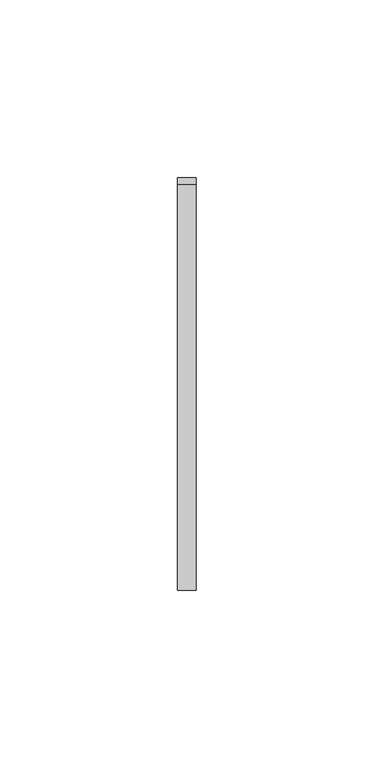
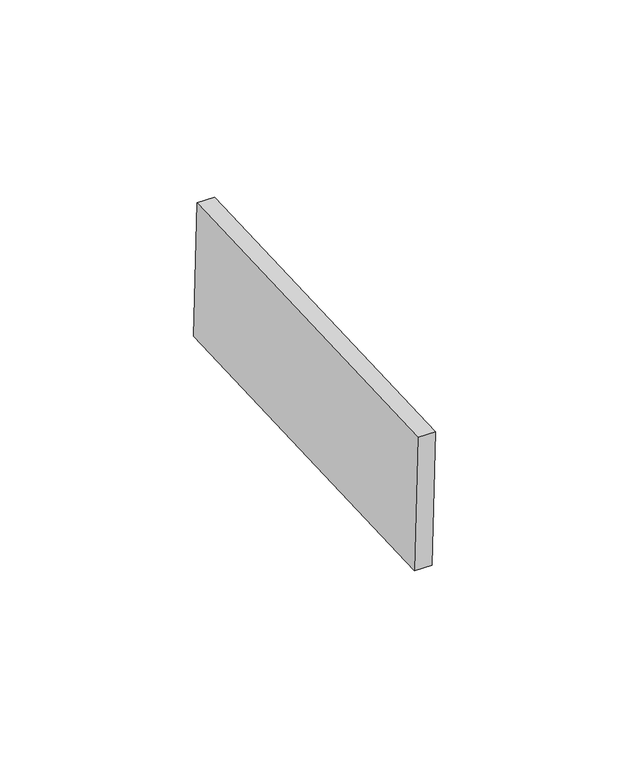
"""IFC4 building model written with IfcOpenShell, lengths in millimetres: proxy geometry, Inner panel:Inner panel:1:Inner panel:1 : Inner panel:Inner panel:300324:2:Inner panel:1:Inner panel:1 : Inner panel:Inner panel:300324:2 : Inner panel:Inner panel:1:Inner panel:1 : Inner panel:Inner panel:300324:300043:84 : Inner panel:Inner panel:1:Inner panel:1 : Inner panel:Inner panel:300324:2:Inner panel:1:Inner panel:1 : Inner panel:Inner panel:300324:2 : Inner panel:Inner panel:1:Inner panel:1 : Inner panel:Inner panel:300324:300043:308120."""

from ifc_helpers import new_model, si_unit, frame, origin, place, context, project, spatial, polyline, outline, extrude, source, transform, mapped, element, save


def generic_models_0b559e5c(model_context):
    return source(origin(), model_context, "Body", "SweptSolid", [
        extrude(outline(polyline([(0.0, -114.2999999), (0.0, 0.0), (5.2138089, 0.0), (5.2138089, -114.2999999), (0.0, -114.2999999)])), frame((593123.795117, -576618.8219505, 4051.6214343), z_axis=(0.0, -0.04163054471216399, 0.9991330730923527), x_axis=(-1.0, 0.0, 0.0)), (0.0, 0.0, 1.0), 43.2233908),
    ])


if __name__ == "__main__":
    model = new_model("IFC4")
    model_context = context("Model", 3, world=origin())
    ifc_project = project(units=[si_unit("LENGTHUNIT", "METRE", prefix="MILLI")], contexts=[model_context])
    site = spatial("IfcSite", under=ifc_project)
    building = spatial("IfcBuilding", under=site)
    placement = place(None, origin())
    generic_models_shape = generic_models_0b559e5c(model_context)
    element("IfcBuildingElementProxy", 1, Name="Inner panel:Inner panel:1:Inner panel:1 : Inner panel:Inner panel:300324:2:Inner panel:1:Inner panel:1 : Inner panel:Inner panel:300324:2 : Inner panel:Inner panel:1:Inner panel:1 : Inner panel:Inner panel:300324:300043:84 : Inner panel:Inner panel:1:Inner panel:1 : Inner panel:Inner panel:300324:2:Inner panel:1:Inner panel:1 : Inner panel:Inner panel:300324:2 : Inner panel:Inner panel:1:Inner panel:1 : Inner panel:Inner panel:300324:300043:308120", ObjectType="Inner panel:Inner panel:1:Inner panel:1 : Inner panel:Inner panel:300324:2:Inner panel:1:Inner panel:1 : Inner panel:Inner panel:300324:2 : Inner panel:Inner panel:1:Inner panel:1 : Inner panel:Inner panel:300324:300043:84 : Inner panel:Inner panel:1:Inner panel:1 : Inner panel:Inner panel:300324:2:Inner panel:1:Inner panel:1 : Inner panel:Inner panel:300324:2 : Inner panel:Inner panel:1:Inner panel:1 : Inner panel:Inner panel:300324:300043:308120", at=placement, inside=building, context=model_context, shape_type="MappedRepresentation", body=[
        mapped(generic_models_shape, transform((0.0, 0.0, 0.0), x_axis=(1.0, 0.0, 0.0), y_axis=(0.0, 1.0, 0.0), z_axis=(0.0, 0.0, 1.0))),
    ])
    save(model, "model.ifc")

# Revit data of these elements
# Type "Inner panel:Inner panel:1:Inner panel:1 : Inner panel:Inner panel:300324:2:Inner panel:1:Inner panel:1 : Inner panel:Inner panel:300324:2 : Inner panel:Inner panel:1:Inner panel:1 : Inner panel:Inner panel:300324:300043:84 : Inner panel:Inner panel:1:Inner panel:1 : Inner panel:Inner panel:300324:2:Inner panel:1:Inner panel:1 : Inner panel:Inner panel:300324:2 : Inner panel:Inner panel:1:Inner panel:1 : Inner panel:Inner panel:300324:300043:308120"
#   NameOverride = "Inner panel:Inner panel:1:Inner panel:1 : Inner panel:Inner panel:300324:2:Inner panel:1:Inner panel:1 : Inner panel:Inner panel:300324:2 : Inner panel:Inner panel:1:Inner panel:1 : Inner panel:Inner panel:300324:300043:308120"
#   ObjectTypeOverride = "Inner panel:1:Inner panel:1 : Inner panel:Inner panel:300324:2 : Inner panel:Inner panel:1:Inner panel:1 : Inner panel:Inner panel:300324:300043"
#   Reference = "Inner panel"
#   Tag = "308120"
# Element 1 (IfcBuildingElementProxy, "Inner panel:Inner panel:1:Inner panel:1 : Inner panel:Inner panel:300324:2:Inner panel:1:Inner panel:1 : Inner panel:Inner panel:300324:2 : Inner panel:Inner panel:1:Inner panel:1 : Inner panel:Inner panel:300324:300043:84 : Inner panel:Inner panel:1:Inner panel:1 : Inner panel:Inner panel:300324:2:Inner panel:1:Inner panel:1 : Inner panel:Inner panel:300324:2 : Inner panel:Inner panel:1:Inner panel:1 : Inner panel:Inner panel:300324:300043:308120")
#   Materials on its faces: "SLIDING CLIP"
# Materials
#   "SLIDING CLIP": class "Generic", colour RGB 120 120 120, transparency 0, Cost = 0
